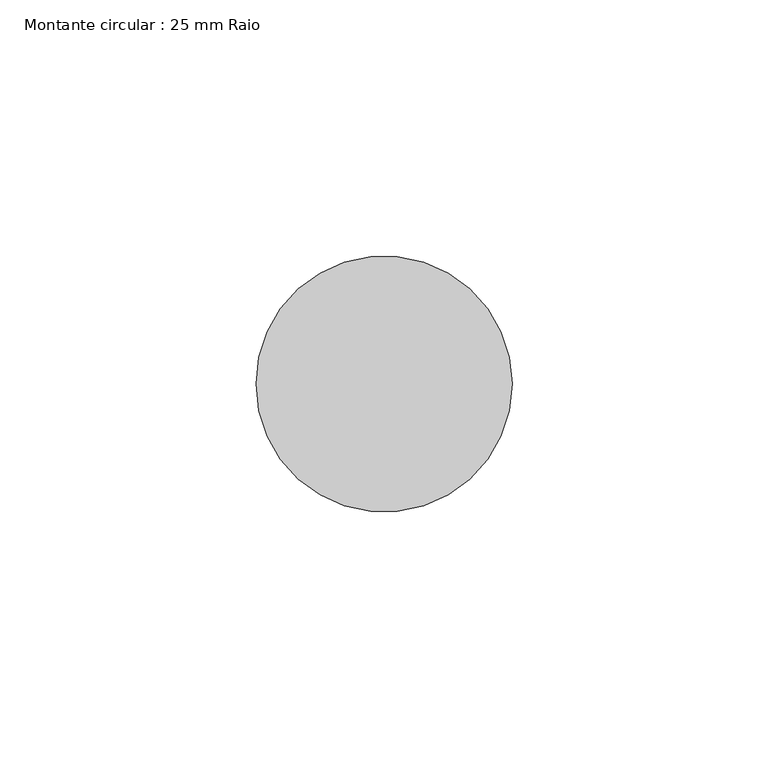
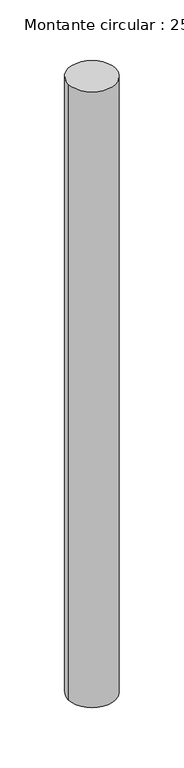
"""IFC4 building model written with IfcOpenShell, lengths in millimetres: member geometry, Montante circular : 25 mm Raio."""

from ifc_helpers import new_model, si_unit, point, frame, frame_2d, origin, place, context, project, spatial, circle_curve, trimmed, segment, composite_curve, outline, extrude, source, transform, mapped, element, save


def montante_circular_25_mm_raio_666f7a7d(model_context):
    return source(origin(), model_context, "Body", "SweptSolid", [
        extrude(outline(composite_curve([segment(trimmed(circle_curve(frame_2d((-25.0, 0.0)), 25.0), [point((0.0, 0.0))], [point((-50.0, 0.0))], False, "CARTESIAN"), True, "CONTINUOUS"), segment(trimmed(circle_curve(frame_2d((-25.0, 0.0)), 25.0), [point((-50.0, 0.0))], [point((0.0, 0.0))], False, "CARTESIAN"), True, "CONTINUOUS")], self_intersect=False)), frame((0.0, 0.0, -685.7133319), z_axis=(0.0, 0.0, 1.0), x_axis=(1.0, 0.0, 0.0)), (0.0, 0.0, 1.0), 685.7133319),
    ])


if __name__ == "__main__":
    model = new_model("IFC4")
    model_context = context("Model", 3, world=origin())
    ifc_project = project(units=[si_unit("LENGTHUNIT", "METRE", prefix="MILLI")], contexts=[model_context])
    site = spatial("IfcSite", under=ifc_project)
    building = spatial("IfcBuilding", under=site)
    placement = place(None, origin())
    montante_circular_25_mm_raio_shape = montante_circular_25_mm_raio_666f7a7d(model_context)
    element("IfcMember", 1, ObjectType="Montante circular : 25 mm Raio", at=placement, inside=building, context=model_context, shape_type="MappedRepresentation", body=[
        mapped(montante_circular_25_mm_raio_shape, transform((0.0, 0.0, 0.0), x_axis=(1.0, 0.0, 0.0), y_axis=(0.0, 1.0, 0.0), z_axis=(0.0, 0.0, 1.0))),
    ])
    save(model, "model.ifc")

# Revit data of these elements
# Type "Montante circular : 25 mm Raio"
#   built-in parameter 1007350 = 0.082021 (stored number, unit not read)
# Element 1 (IfcMember, "Montante circular : 25 mm Raio")
#   Materials on its faces: "Alumín."
# Materials
#   "Alumín.": class "Metal", colour RGB 247 247 247, transparency 0, Description = "Alumín. 6061", Cost = 0
